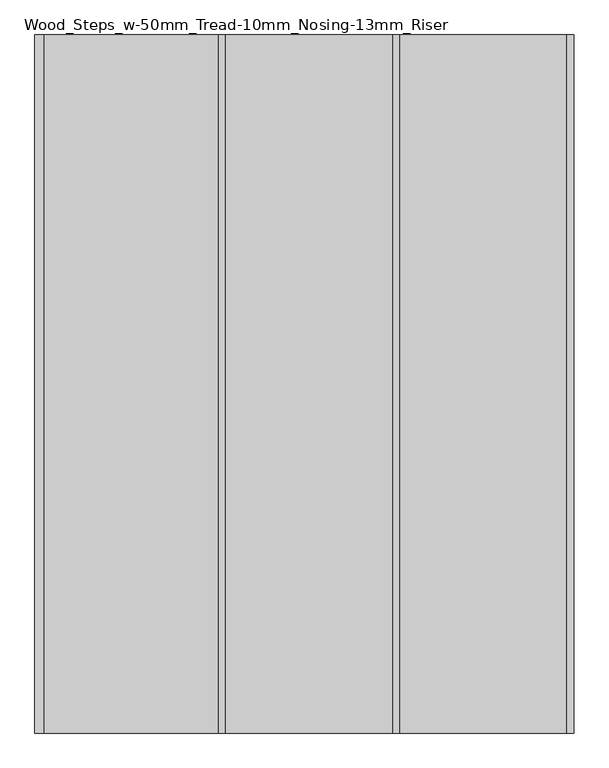
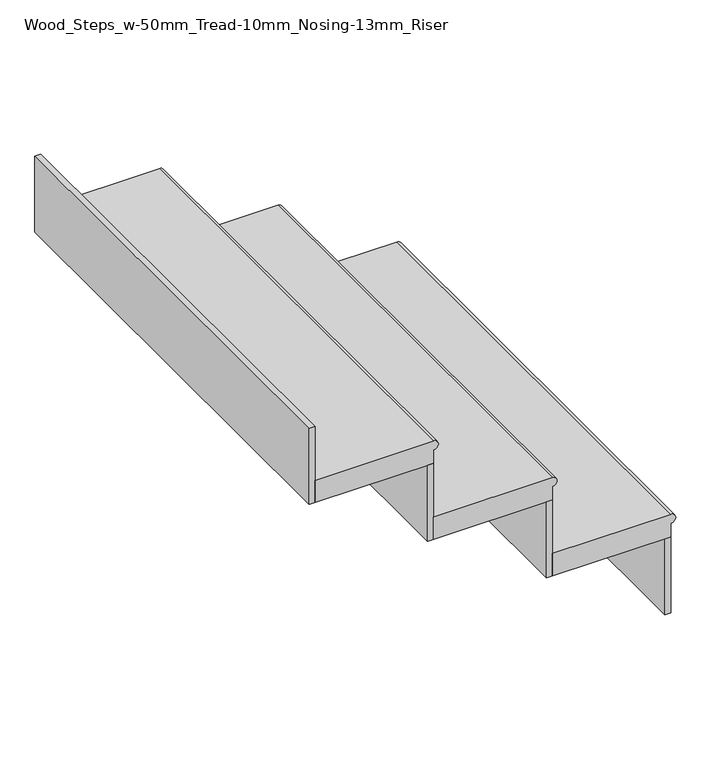
"""IFC4 building model written with IfcOpenShell, lengths in millimetres: stair flight geometry, Wood_Steps_w-50mm_Tread-10mm_Nosing-13mm_Riser."""

from ifc_helpers import new_model, si_unit, point, frame, frame_2d, origin, place, context, project, spatial, polyline, circle_curve, trimmed, segment, composite_curve, outline, extrude, source, transform, mapped, element, save


def wood_steps_w_50mm_tread_10mm_nosing_13mm_riser_8e23bed2(model_context):
    return source(origin(), model_context, "Body", "SweptSolid", [
        extrude(outline(composite_curve([segment(polyline([(2819.6235294, 2406.940348), (2819.6235294, 2156.940348), (2769.6235294, 2156.940348), (2769.6235294, 2406.940348), (2799.6235294, 2406.940348)]), True, "CONTINUOUS"), segment(trimmed(circle_curve(frame_2d((2809.6235294, 2406.940348)), 10.0), [point((2799.6235294, 2406.940348))], [point((2819.6235294, 2406.940348))], False, "CARTESIAN"), True, "CONTINUOUS")], self_intersect=False)), frame((0.0, 1631.1308056, 0.0), z_axis=(0.0, 1.0, 0.0), x_axis=(0.0, 0.0, 1.0)), (0.0, 0.0, 1.0), 1000.0),
        extrude(outline(polyline([(2394.440348, 2631.1308056), (2406.940348, 2631.1308056), (2406.940348, 1631.1308056), (2394.440348, 1631.1308056), (2394.440348, 2631.1308056)])), frame((0.0, 0.0, 2600.3647059), z_axis=(0.0, 0.0, 1.0), x_axis=(1.0, 0.0, 0.0)), (0.0, 0.0, 1.0), 169.2588235),
        extrude(outline(polyline([(2144.440348, 2631.1308056), (2156.940348, 2631.1308056), (2156.940348, 1631.1308056), (2144.440348, 1631.1308056), (2144.440348, 2631.1308056)])), frame((0.0, 0.0, 2769.6235294), z_axis=(0.0, 0.0, 1.0), x_axis=(1.0, 0.0, 0.0)), (0.0, 0.0, 1.0), 169.2588235),
        extrude(outline(composite_curve([segment(polyline([(2988.8823529, 2156.940348), (2988.8823529, 1906.940348), (2938.8823529, 1906.940348), (2938.8823529, 2156.940348), (2968.8823529, 2156.940348)]), True, "CONTINUOUS"), segment(trimmed(circle_curve(frame_2d((2978.8823529, 2156.940348)), 10.0), [point((2968.8823529, 2156.940348))], [point((2988.8823529, 2156.940348))], False, "CARTESIAN"), True, "CONTINUOUS")], self_intersect=False)), frame((0.0, 1631.1308056, 0.0), z_axis=(0.0, 1.0, 0.0), x_axis=(0.0, 0.0, 1.0)), (0.0, 0.0, 1.0), 1000.0),
        extrude(outline(polyline([(1894.440348, 2631.1308056), (1906.940348, 2631.1308056), (1906.940348, 1631.1308056), (1894.440348, 1631.1308056), (1894.440348, 2631.1308056)])), frame((0.0, 0.0, 2938.8823529), z_axis=(0.0, 0.0, 1.0), x_axis=(1.0, 0.0, 0.0)), (0.0, 0.0, 1.0), 169.2588235),
        extrude(outline(polyline([(1644.440348, 2631.1308056), (1656.940348, 2631.1308056), (1656.940348, 1631.1308056), (1644.440348, 1631.1308056), (1644.440348, 2631.1308056)])), frame((0.0, 0.0, 3108.1411765), z_axis=(0.0, 0.0, 1.0), x_axis=(1.0, 0.0, 0.0)), (0.0, 0.0, 1.0), 169.2588235),
        extrude(outline(composite_curve([segment(polyline([(3158.1411765, 1906.940348), (3158.1411765, 1656.940348), (3108.1411765, 1656.940348), (3108.1411765, 1906.940348), (3138.1411765, 1906.940348)]), True, "CONTINUOUS"), segment(trimmed(circle_curve(frame_2d((3148.1411765, 1906.940348)), 10.0), [point((3138.1411765, 1906.940348))], [point((3158.1411765, 1906.940348))], False, "CARTESIAN"), True, "CONTINUOUS")], self_intersect=False)), frame((0.0, 1631.1308056, 0.0), z_axis=(0.0, 1.0, 0.0), x_axis=(0.0, 0.0, 1.0)), (0.0, 0.0, 1.0), 1000.0),
    ])


if __name__ == "__main__":
    model = new_model("IFC4")
    model_context = context("Model", 3, world=origin())
    ifc_project = project(units=[si_unit("LENGTHUNIT", "METRE", prefix="MILLI")], contexts=[model_context])
    site = spatial("IfcSite", under=ifc_project)
    building = spatial("IfcBuilding", under=site)
    placement = place(None, origin())
    wood_steps_w_50mm_tread_10mm_nosing_13mm_riser_shape = wood_steps_w_50mm_tread_10mm_nosing_13mm_riser_8e23bed2(model_context)
    element("IfcStairFlight", 1, ObjectType="Wood_Steps_w-50mm_Tread-10mm_Nosing-13mm_Riser", at=placement, inside=building, context=model_context, shape_type="MappedRepresentation", body=[
        mapped(wood_steps_w_50mm_tread_10mm_nosing_13mm_riser_shape, transform((0.0, 0.0, 0.0), x_axis=(1.0, 0.0, 0.0), y_axis=(0.0, 1.0, 0.0), z_axis=(0.0, 0.0, 1.0))),
    ])
    save(model, "model.ifc")

# Revit data of these elements
# Element 1 (IfcStairFlight, "Wood_Steps_w-50mm_Tread-10mm_Nosing-13mm_Riser")
#   Materials on its faces: "Oak Flooring"
# Materials
#   "Oak Flooring": class "Wood", colour RGB 212 179 113, transparency 0, Description = "Quercus Rubra", Cost = 0
